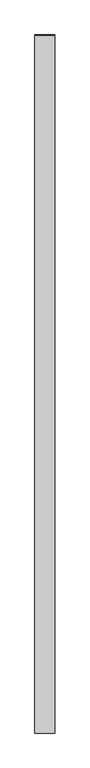
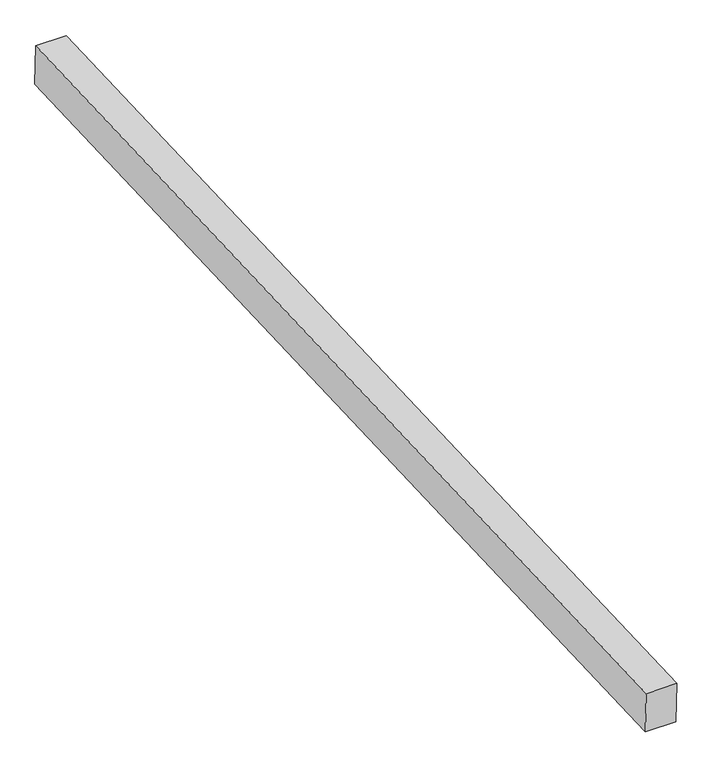
"""IFC4 building model written with IfcOpenShell, lengths in millimetres: proxy geometry, Generic Models 7:Generic Models 1:8:Generic Models 1:8 : Generic Models 7:Generic Models 1:337419:38 : Generic Models 7:Generic Models 1:8:Generic Models 1:8 : Generic Models 7:Generic Models 1:337419:315935."""

from ifc_helpers import new_model, si_unit, frame, origin, place, context, project, spatial, polyline, outline, extrude, source, transform, mapped, element, save


def generic_models_70ed6090(model_context):
    return source(origin(), model_context, "Body", "SweptSolid", [
        extrude(outline(polyline([(-581229.2495411, 3818.908703), (-576356.3266468, 4021.9471569), (-576348.7597251, 3831.5971524), (-581221.3189223, 3628.5738526), (-581229.2495411, 3818.908703)])), frame((664746.9617239, 0.0, 0.0), z_axis=(1.0, 0.0, 0.0), x_axis=(0.0, 1.0, 0.0)), (0.0, 0.0, 1.0), 139.7),
    ])


if __name__ == "__main__":
    model = new_model("IFC4")
    model_context = context("Model", 3, world=origin())
    ifc_project = project(units=[si_unit("LENGTHUNIT", "METRE", prefix="MILLI")], contexts=[model_context])
    site = spatial("IfcSite", under=ifc_project)
    building = spatial("IfcBuilding", under=site)
    placement = place(None, origin())
    generic_models_shape = generic_models_70ed6090(model_context)
    element("IfcBuildingElementProxy", 1, Name="Generic Models 7:Generic Models 1:8:Generic Models 1:8 : Generic Models 7:Generic Models 1:337419:38 : Generic Models 7:Generic Models 1:8:Generic Models 1:8 : Generic Models 7:Generic Models 1:337419:315935", ObjectType="Generic Models 7:Generic Models 1:8:Generic Models 1:8 : Generic Models 7:Generic Models 1:337419:38 : Generic Models 7:Generic Models 1:8:Generic Models 1:8 : Generic Models 7:Generic Models 1:337419:315935", at=placement, inside=building, context=model_context, shape_type="MappedRepresentation", body=[
        mapped(generic_models_shape, transform((0.0, 0.0, 0.0), x_axis=(1.0, 0.0, 0.0), y_axis=(0.0, 1.0, 0.0), z_axis=(0.0, 0.0, 1.0))),
    ])
    save(model, "model.ifc")

# Revit data of these elements
# Type "Generic Models 7:Generic Models 1:8:Generic Models 1:8 : Generic Models 7:Generic Models 1:337419:38 : Generic Models 7:Generic Models 1:8:Generic Models 1:8 : Generic Models 7:Generic Models 1:337419:315935"
#   NameOverride = "Generic Models 7:Generic Models 1:8:Generic Models 1:8 : Generic Models 7:Generic Models 1:337419:315935"
#   ObjectTypeOverride = "Generic Models 1:8 : Generic Models 7:Generic Models 1:337419"
#   Reference = "Generic Models 1"
#   Tag = "315935"
# Element 1 (IfcBuildingElementProxy, "Generic Models 7:Generic Models 1:8:Generic Models 1:8 : Generic Models 7:Generic Models 1:337419:38 : Generic Models 7:Generic Models 1:8:Generic Models 1:8 : Generic Models 7:Generic Models 1:337419:315935")
#   Materials on its faces: "5 1/2\" X 7 1/2\" EXTERIOR GRADE GLULAM BEAMS"
# Materials
#   "5 1/2\" X 7 1/2\" EXTERIOR GRADE GLULAM BEAMS": class "Wood", colour RGB 183 134 68, transparency 0, Keynote = "M06181300.01", Description = "Pinus Echinata", Cost = 0
